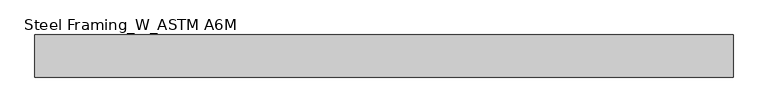
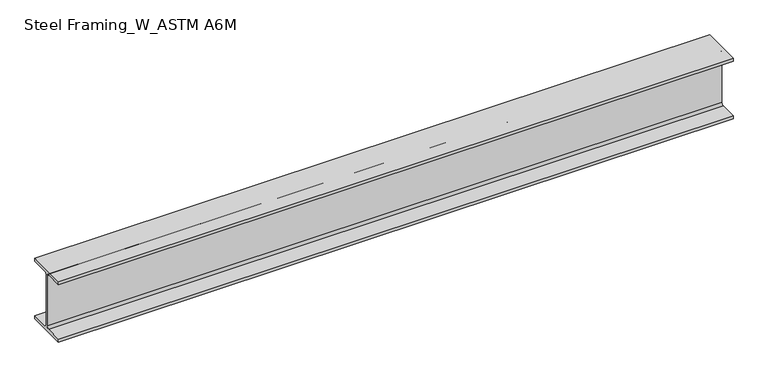
"""IFC4 building model written with IfcOpenShell, lengths in millimetres: beam geometry, Steel Framing_W_ASTM A6M : H_SB_AR_S02_W200x31.3_B6."""

from ifc_helpers import new_model, si_unit, point, frame, frame_2d, origin, place, context, project, spatial, polyline, circle_curve, trimmed, segment, composite_curve, outline, extrude, source, transform, mapped, element, save


def steel_framing_w_astm_a6m_4302fd06(model_context):
    return source(origin(), model_context, "Body", "SweptSolid", [
        extrude(outline(composite_curve([segment(polyline([(67.0, -94.8), (67.0, -105.0), (-67.0, -105.0), (-67.0, -94.8), (-10.775, -94.8)]), True, "CONTINUOUS"), segment(trimmed(circle_curve(frame_2d((-10.775, -87.2)), 7.6), [point((-10.775, -94.8))], [point((-3.175, -87.2))], True, "CARTESIAN"), True, "CONTINUOUS"), segment(polyline([(-3.175, -87.2), (-3.175, 87.2)]), True, "CONTINUOUS"), segment(trimmed(circle_curve(frame_2d((-10.775, 87.2)), 7.6), [point((-3.175, 87.2))], [point((-10.775, 94.8))], True, "CARTESIAN"), True, "CONTINUOUS"), segment(polyline([(-10.775, 94.8), (-67.0, 94.8), (-67.0, 105.0), (67.0, 105.0), (67.0, 94.8), (10.775, 94.8)]), True, "CONTINUOUS"), segment(trimmed(circle_curve(frame_2d((10.775, 87.2)), 7.6), [point((10.775, 94.8))], [point((3.175, 87.2))], True, "CARTESIAN"), True, "CONTINUOUS"), segment(polyline([(3.175, 87.2), (3.175, -87.2)]), True, "CONTINUOUS"), segment(trimmed(circle_curve(frame_2d((10.775, -87.2)), 7.6), [point((3.175, -87.2))], [point((10.775, -94.8))], True, "CARTESIAN"), True, "CONTINUOUS"), segment(polyline([(10.775, -94.8), (67.0, -94.8)]), True, "CONTINUOUS")], self_intersect=False)), frame((-1151.8, 0.0, 0.0), z_axis=(1.0, 0.0, 0.0), x_axis=(0.0, 1.0, 0.0)), (0.0, 0.0, 1.0), 2220.9),
    ])


if __name__ == "__main__":
    model = new_model("IFC4")
    model_context = context("Model", 3, world=origin())
    ifc_project = project(units=[si_unit("LENGTHUNIT", "METRE", prefix="MILLI")], contexts=[model_context])
    site = spatial("IfcSite", under=ifc_project)
    building = spatial("IfcBuilding", under=site)
    placement = place(None, origin())
    steel_framing_w_astm_a6m_shape = steel_framing_w_astm_a6m_4302fd06(model_context)
    element("IfcBeam", 1, ObjectType="Steel Framing_W_ASTM A6M : H_SB_AR_S02_W200x31.3_B6", at=placement, inside=building, context=model_context, shape_type="MappedRepresentation", body=[
        mapped(steel_framing_w_astm_a6m_shape, transform((0.0, 0.0, 0.0), x_axis=(1.0, 0.0, 0.0), y_axis=(0.0, 1.0, 0.0), z_axis=(0.0, 0.0, 1.0))),
    ])
    save(model, "model.ifc")

# Revit data of these elements
# Type "Steel Framing_W_ASTM A6M : H_SB_AR_S02_W200x31.3_B6"
#   Type Mark = "B6"
#   Section Name Key = "W8x21"
#   Width = 13.4 cm
#   Web Thickness = 0.635 cm
#   Web Fillet = 0.76 cm
#   Warping Constant = 40800.0 cm⁶
#   Torsional Moment of Inertia = 11.70 cm⁴
#   Section Area = 39.7 cm²
#   Plastic Modulus weak axis = 93.2 cm³
#   Plastic Modulus strong axis = 334.0 cm³
#   Perimeter = 0.93 m²/m
#   Nominal Weight = 31.30 kgf/m
#   Moment of Inertia weak axis = 407.00 cm⁴
#   Moment of Inertia strong axis = 3130.00 cm⁴
#   Height = 21.0 cm
#   Flange Thickness = 1.02 cm
#   Elastic Modulus weak axis = 60.8 cm³
#   Elastic Modulus strong axis = 298.0 cm³
#   Centroid Vertical = 10.5 cm
#   Centroid Horizontal = 6.7 cm
#   Length [instance default] = 1500 mm
#   Structural Material [instance default] = Steel, 45-345
#   Bolt Spacing = 0
#   Assembly Code = ""
# Element 1 (IfcBeam, "Steel Framing_W_ASTM A6M : H_SB_AR_S02_W200x31.3_B6")
#   Materials on its faces: "Steel, 45-345"
# Materials
#   "Steel, 45-345": class "Metal", colour RGB 189 187 185, transparency 0, Description = "Steel 345 MPa", Cost = 0
